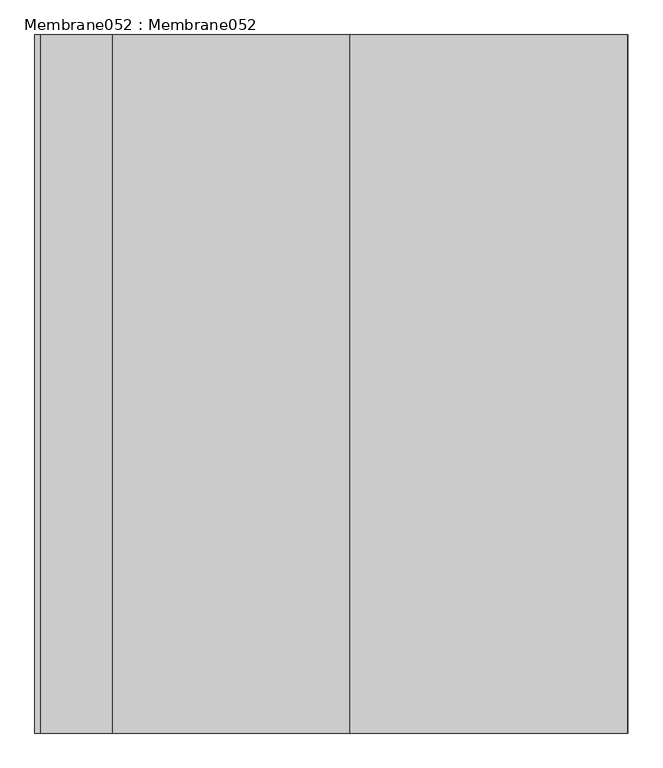
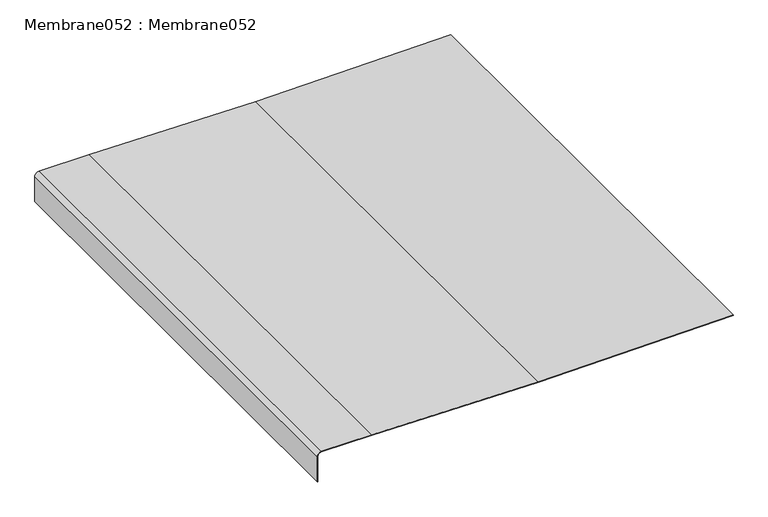
"""IFC4 building model written with IfcOpenShell, lengths in millimetres: proxy geometry, Membrane052 : Membrane052."""

import ifcopenshell
import ifcopenshell.guid

model = None  # the IFC model being written
_history = None  # IfcOwnerHistory: only IFC2X3 demands one
_inside = {}  # id of a spatial element -> (the spatial element, [elements in it])
_under = {}  # id of a project, library or spatial element -> (it, [spatial elements below it])
_declared = {}  # id of a project -> (the project, [libraries it declares])
_typed = {}  # id of a type object -> (the type object, [elements of that type])
_made_of = {}  # id of a material, layer set ... -> (it, [elements and type objects made of it])


def new_model(schema):
    """Start an empty IFC model of exactly this schema.

    Asked for "IFC4X3", IfcOpenShell would pick the latest addendum, in which some entities
    have other attributes; the version numbers below select the first issue.
    IFC2X3 requires an IfcOwnerHistory on every rooted entity: one is made here for all.
    """
    global model, _history
    if schema == "IFC4X3":
        model = ifcopenshell.file(schema_version=(4, 3, 0, 0))
    else:
        model = ifcopenshell.file(schema=schema)
    _inside.clear()
    _under.clear()
    _declared.clear()
    _typed.clear()
    _made_of.clear()
    _history = None
    if model.schema == "IFC2X3":
        org = make("IfcOrganization", Name="unknown")
        user = make(
            "IfcPersonAndOrganization",
            ThePerson=make("IfcPerson", FamilyName="unknown"),
            TheOrganization=org,
        )
        app = make(
            "IfcApplication",
            ApplicationDeveloper=org,
            Version="unknown",
            ApplicationFullName="unknown",
            ApplicationIdentifier="unknown",
        )
        _history = make(
            "IfcOwnerHistory",
            OwningUser=user,
            OwningApplication=app,
            ChangeAction="ADDED",
            CreationDate=0,
        )
    return model


def make(cls, **values):
    """One entity of the class cls with the attributes given. An attribute that is None is left unset."""
    return model.create_entity(
        cls, **{name: value for name, value in values.items() if value is not None}
    )


def rooted(cls, **values):
    """An entity with a GlobalId (a new one), such as an element, a storey or a relation."""
    return make(cls, GlobalId=ifcopenshell.guid.new(), OwnerHistory=_history, **values)


def si_unit(unit_type, name, prefix=None):
    """IfcSIUnit, for example si_unit("LENGTHUNIT", "METRE", prefix="MILLI")."""
    return make("IfcSIUnit", UnitType=unit_type, Prefix=prefix, Name=name)


def assignment(units):
    """IfcUnitAssignment: the units of a project."""
    return None if units is None else make("IfcUnitAssignment", Units=units)


def point(xyz):
    """IfcCartesianPoint."""
    return None if xyz is None else make("IfcCartesianPoint", Coordinates=xyz)


def direction(xyz):
    """IfcDirection."""
    return None if xyz is None else make("IfcDirection", DirectionRatios=xyz)


def frame(location, z_axis=None, x_axis=None):
    """IfcAxis2Placement3D, a coordinate frame: its origin and axes. An axis left out is left unset."""
    return make(
        "IfcAxis2Placement3D",
        Location=point(location),
        Axis=direction(z_axis),
        RefDirection=direction(x_axis),
    )


def frame_2d(location, x_axis=None):
    """IfcAxis2Placement2D, a coordinate frame in the plane: its origin and x axis."""
    return make(
        "IfcAxis2Placement2D", Location=point(location), RefDirection=direction(x_axis)
    )


def origin():
    """The frame at (0, 0, 0) with its axes left unset."""
    return frame((0.0, 0.0, 0.0))


def place(relative_to, where):
    """IfcLocalPlacement: puts the frame where relative to a parent placement (None: the world)."""
    return make(
        "IfcLocalPlacement", PlacementRelTo=relative_to, RelativePlacement=where
    )


def context(
    kind, dimensions, precision=None, world=None, true_north=None, identifier=None
):
    """IfcGeometricRepresentationContext, for example the 3D "Model" context."""
    return make(
        "IfcGeometricRepresentationContext",
        ContextIdentifier=identifier,
        ContextType=kind,
        CoordinateSpaceDimension=dimensions,
        Precision=precision,
        WorldCoordinateSystem=world,
        TrueNorth=true_north,
    )


def project(units=None, contexts=None):
    """IfcProject with its units and contexts."""
    return rooted(
        "IfcProject",
        Name="project",
        RepresentationContexts=contexts,
        UnitsInContext=assignment(units),
    )


def spatial(cls, under=None, at=None, **own):
    """A site, building, storey or space (cls), placed at a placement, below another one or the project."""
    s = rooted(cls, ObjectPlacement=at, **own)
    if under is not None:
        _under.setdefault(under.id(), (under, []))[1].append(s)
    return s


def polyline(points):
    """IfcPolyline through the points."""
    return make("IfcPolyline", Points=[point(p) for p in points])


def circle_curve(where, radius):
    """IfcCircle in the frame where."""
    return make("IfcCircle", Position=where, Radius=radius)


def trimmed(basis, trim1, trim2, sense, master):
    """IfcTrimmedCurve: the piece of a basis curve between two trims."""
    return make(
        "IfcTrimmedCurve",
        BasisCurve=basis,
        Trim1=trim1,
        Trim2=trim2,
        SenseAgreement=sense,
        MasterRepresentation=master,
    )


def segment(curve, same_sense, transition):
    """IfcCompositeCurveSegment."""
    return make(
        "IfcCompositeCurveSegment",
        Transition=transition,
        SameSense=same_sense,
        ParentCurve=curve,
    )


def composite_curve(segments, self_intersect=None):
    """IfcCompositeCurve: segments joined end to end."""
    return make("IfcCompositeCurve", Segments=segments, SelfIntersect=self_intersect)


def outline(outer, holes=None, kind="AREA"):
    """IfcArbitraryClosedProfileDef: a profile drawn as a closed curve; with holes, ...WithVoids."""
    if holes is None:
        return make("IfcArbitraryClosedProfileDef", ProfileType=kind, OuterCurve=outer)
    return make(
        "IfcArbitraryProfileDefWithVoids",
        ProfileType=kind,
        OuterCurve=outer,
        InnerCurves=holes,
    )


def extrude(swept, where, along, depth):
    """IfcExtrudedAreaSolid: the profile swept, set in the frame where, extruded along a direction by depth."""
    return make(
        "IfcExtrudedAreaSolid",
        SweptArea=swept,
        Position=where,
        ExtrudedDirection=direction(along),
        Depth=depth,
    )


def shape(context_of_items, identifier, shape_type, items):
    """IfcShapeRepresentation: the items that make up one representation, for example the "Body"."""
    return make(
        "IfcShapeRepresentation",
        ContextOfItems=context_of_items,
        RepresentationIdentifier=identifier,
        RepresentationType=shape_type,
        Items=items,
    )


def source(mapping_origin, context_of_items, identifier, shape_type, items):
    """IfcRepresentationMap: a shape defined once, which mapped items show again and again."""
    return make(
        "IfcRepresentationMap",
        MappingOrigin=mapping_origin,
        MappedRepresentation=shape(context_of_items, identifier, shape_type, items),
    )


def transform(
    local_origin,
    x_axis=None,
    y_axis=None,
    z_axis=None,
    scale=None,
    scale2=None,
    scale3=None,
    uniform=True,
):
    """IfcCartesianTransformationOperator3D, or its non-uniform kind. x_axis, y_axis, z_axis: its Axis1, 2, 3."""
    if uniform:
        return make(
            "IfcCartesianTransformationOperator3D",
            Axis1=direction(x_axis),
            Axis2=direction(y_axis),
            LocalOrigin=point(local_origin),
            Scale=scale,
            Axis3=direction(z_axis),
        )
    return make(
        "IfcCartesianTransformationOperator3DnonUniform",
        Axis1=direction(x_axis),
        Axis2=direction(y_axis),
        LocalOrigin=point(local_origin),
        Scale=scale,
        Axis3=direction(z_axis),
        Scale2=scale2,
        Scale3=scale3,
    )


def mapped(mapping_source, mapping_target):
    """IfcMappedItem: shows the shape of a source again, moved by a transform."""
    return make(
        "IfcMappedItem", MappingSource=mapping_source, MappingTarget=mapping_target
    )


def made_of(thing, what):
    """Note that an element or type object is made of a material, layer set ...; save() writes the relation."""
    if what is not None:
        _made_of.setdefault(what.id(), (what, []))[1].append(thing)
    return thing


def element(
    cls,
    number,
    at=None,
    inside=None,
    cuts=None,
    type_object=None,
    material=None,
    context=None,
    identifier="Body",
    shape_type=None,
    held_by="IfcProductDefinitionShape",
    body=None,
    shapes=None,
    **own,
):
    """One element of the class cls, such as IfcWall. Its Tag is "e" and its number.

    at: its placement. inside: the storey or other place that contains it. cuts: it is an
    opening in that element (IfcRelVoidsElement). A single representation is given by context,
    identifier, shape_type and body (its items); several are given by shapes. held_by: the class
    of the entity that holds the representations. save() writes the other relations.
    """
    e = rooted(cls, Tag="e%d" % number, ObjectPlacement=at, **own)
    if body is not None:
        shapes = [shape(context, identifier, shape_type, body)]
    if shapes is not None:
        e.Representation = make(held_by, Representations=shapes)
    if inside is not None:
        _inside.setdefault(inside.id(), (inside, []))[1].append(e)
    if cuts is not None:
        rooted(
            "IfcRelVoidsElement", RelatingBuildingElement=cuts, RelatedOpeningElement=e
        )
    if type_object is not None:
        _typed.setdefault(type_object.id(), (type_object, []))[1].append(e)
    return made_of(e, material)


def aggregate(whole, parts):
    """IfcRelAggregates: a whole, such as a stair, and the parts it consists of."""
    return rooted("IfcRelAggregates", RelatingObject=whole, RelatedObjects=parts)


def save(model, path):
    """Write the relations noted so far, then the file.

    IfcRelAggregates (storeys below a building ...), IfcRelContainedInSpatialStructure (elements
    in a storey), IfcRelDefinesByType, IfcRelAssociatesMaterial and IfcRelDeclares: one each for
    every whole, place, type object, material and project.
    """
    for whole, parts in _under.values():
        aggregate(whole, parts)
    for where, things in _inside.values():
        rooted(
            "IfcRelContainedInSpatialStructure",
            RelatedElements=things,
            RelatingStructure=where,
        )
    for kind, things in _typed.values():
        rooted("IfcRelDefinesByType", RelatedObjects=things, RelatingType=kind)
    for what, things in _made_of.values():
        rooted("IfcRelAssociatesMaterial", RelatedObjects=things, RelatingMaterial=what)
    for by, libraries in _declared.values():
        rooted("IfcRelDeclares", RelatingContext=by, RelatedDefinitions=libraries)
    model.write(path)


def membrane052_membrane052_5c073de5(model_context):
    return source(origin(), model_context, "Body", "SweptSolid", [
        extrude(outline(composite_curve([segment(trimmed(circle_curve(frame_2d((40234.8417335, -2783.0546039)), 15.0), [point((40234.8417335, -2798.0546039))], [point((40249.8417335, -2783.0546039))], True, "CARTESIAN"), True, "CONTINUOUS"), segment(polyline([(40249.8417335, -2783.0546039), (40249.8417335, -2577.3779567), (40240.0438802, -1896.5672037), (40249.8417335, -1100.0857963), (40251.8415822, -1100.1103973), (40242.0440572, -1896.5651139), (40251.8417335, -2577.3635659), (40251.8417335, -2783.0546039)]), True, "CONTINUOUS"), segment(trimmed(circle_curve(frame_2d((40234.8417335, -2783.0546039)), 17.0), [point((40251.8417335, -2783.0546039))], [point((40234.8417335, -2800.0546039))], False, "CARTESIAN"), True, "CONTINUOUS"), segment(polyline([(40234.8417335, -2800.0546039), (40125.2457074, -2800.0546039), (40125.2457074, -2798.0546039), (40234.8417335, -2798.0546039)]), True, "CONTINUOUS")], self_intersect=False)), frame((0.0, -1052.8906574, 0.0), z_axis=(0.0, 1.0, 0.0), x_axis=(0.0, 0.0, 1.0)), (0.0, 0.0, 1.0), 2000.0),
    ])


if __name__ == "__main__":
    model = new_model("IFC4")
    model_context = context("Model", 3, world=origin())
    ifc_project = project(units=[si_unit("LENGTHUNIT", "METRE", prefix="MILLI")], contexts=[model_context])
    site = spatial("IfcSite", under=ifc_project)
    building = spatial("IfcBuilding", under=site)
    placement = place(None, origin())
    membrane052_membrane052_shape = membrane052_membrane052_5c073de5(model_context)
    element("IfcBuildingElementProxy", 1, Name="Membrane052 : Membrane052", ObjectType="Membrane052 : Membrane052", at=placement, inside=building, context=model_context, shape_type="MappedRepresentation", body=[
        mapped(membrane052_membrane052_shape, transform((0.0, 0.0, 0.0), x_axis=(1.0, 0.0, 0.0), y_axis=(0.0, 1.0, 0.0), z_axis=(0.0, 0.0, 1.0))),
    ])
    save(model, "model.ifc")

# Revit data of these elements
# Type "Membrane052 : Membrane052"
#   NameOverride = "Membrane052"
# Element 1 (IfcBuildingElementProxy, "Membrane052 : Membrane052")
#   Materials on its faces: "THREE PLY BUILT UP ROOF MEMBRANE"
# Materials
#   "THREE PLY BUILT UP ROOF MEMBRANE": class "Unassigned", colour RGB 63 63 63, transparency 0
